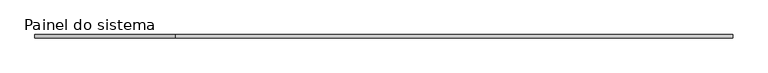
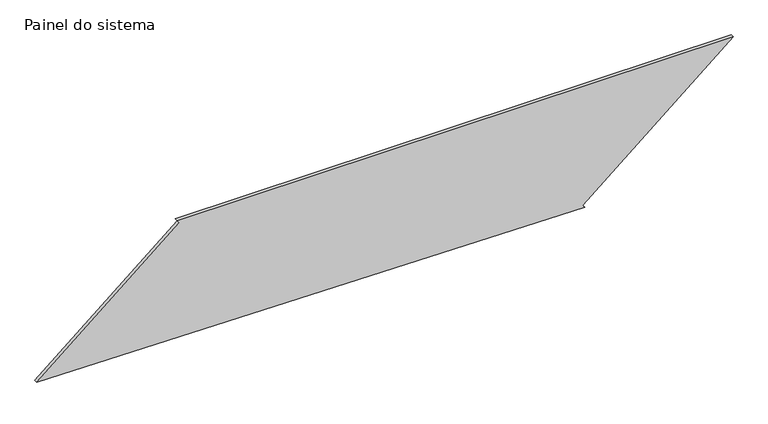
"""IFC4 building model written with IfcOpenShell, lengths in millimetres: plate geometry, Painel do sistema : Envidraçado."""

import ifcopenshell
import ifcopenshell.guid

model = None  # the IFC model being written
_history = None  # IfcOwnerHistory: only IFC2X3 demands one
_inside = {}  # id of a spatial element -> (the spatial element, [elements in it])
_under = {}  # id of a project, library or spatial element -> (it, [spatial elements below it])
_declared = {}  # id of a project -> (the project, [libraries it declares])
_typed = {}  # id of a type object -> (the type object, [elements of that type])
_made_of = {}  # id of a material, layer set ... -> (it, [elements and type objects made of it])


def new_model(schema):
    """Start an empty IFC model of exactly this schema.

    Asked for "IFC4X3", IfcOpenShell would pick the latest addendum, in which some entities
    have other attributes; the version numbers below select the first issue.
    IFC2X3 requires an IfcOwnerHistory on every rooted entity: one is made here for all.
    """
    global model, _history
    if schema == "IFC4X3":
        model = ifcopenshell.file(schema_version=(4, 3, 0, 0))
    else:
        model = ifcopenshell.file(schema=schema)
    _inside.clear()
    _under.clear()
    _declared.clear()
    _typed.clear()
    _made_of.clear()
    _history = None
    if model.schema == "IFC2X3":
        org = make("IfcOrganization", Name="unknown")
        user = make(
            "IfcPersonAndOrganization",
            ThePerson=make("IfcPerson", FamilyName="unknown"),
            TheOrganization=org,
        )
        app = make(
            "IfcApplication",
            ApplicationDeveloper=org,
            Version="unknown",
            ApplicationFullName="unknown",
            ApplicationIdentifier="unknown",
        )
        _history = make(
            "IfcOwnerHistory",
            OwningUser=user,
            OwningApplication=app,
            ChangeAction="ADDED",
            CreationDate=0,
        )
    return model


def make(cls, **values):
    """One entity of the class cls with the attributes given. An attribute that is None is left unset."""
    return model.create_entity(
        cls, **{name: value for name, value in values.items() if value is not None}
    )


def rooted(cls, **values):
    """An entity with a GlobalId (a new one), such as an element, a storey or a relation."""
    return make(cls, GlobalId=ifcopenshell.guid.new(), OwnerHistory=_history, **values)


def si_unit(unit_type, name, prefix=None):
    """IfcSIUnit, for example si_unit("LENGTHUNIT", "METRE", prefix="MILLI")."""
    return make("IfcSIUnit", UnitType=unit_type, Prefix=prefix, Name=name)


def assignment(units):
    """IfcUnitAssignment: the units of a project."""
    return None if units is None else make("IfcUnitAssignment", Units=units)


def point(xyz):
    """IfcCartesianPoint."""
    return None if xyz is None else make("IfcCartesianPoint", Coordinates=xyz)


def direction(xyz):
    """IfcDirection."""
    return None if xyz is None else make("IfcDirection", DirectionRatios=xyz)


def frame(location, z_axis=None, x_axis=None):
    """IfcAxis2Placement3D, a coordinate frame: its origin and axes. An axis left out is left unset."""
    return make(
        "IfcAxis2Placement3D",
        Location=point(location),
        Axis=direction(z_axis),
        RefDirection=direction(x_axis),
    )


def origin():
    """The frame at (0, 0, 0) with its axes left unset."""
    return frame((0.0, 0.0, 0.0))


def place(relative_to, where):
    """IfcLocalPlacement: puts the frame where relative to a parent placement (None: the world)."""
    return make(
        "IfcLocalPlacement", PlacementRelTo=relative_to, RelativePlacement=where
    )


def context(
    kind, dimensions, precision=None, world=None, true_north=None, identifier=None
):
    """IfcGeometricRepresentationContext, for example the 3D "Model" context."""
    return make(
        "IfcGeometricRepresentationContext",
        ContextIdentifier=identifier,
        ContextType=kind,
        CoordinateSpaceDimension=dimensions,
        Precision=precision,
        WorldCoordinateSystem=world,
        TrueNorth=true_north,
    )


def project(units=None, contexts=None):
    """IfcProject with its units and contexts."""
    return rooted(
        "IfcProject",
        Name="project",
        RepresentationContexts=contexts,
        UnitsInContext=assignment(units),
    )


def spatial(cls, under=None, at=None, **own):
    """A site, building, storey or space (cls), placed at a placement, below another one or the project."""
    s = rooted(cls, ObjectPlacement=at, **own)
    if under is not None:
        _under.setdefault(under.id(), (under, []))[1].append(s)
    return s


def polyline(points):
    """IfcPolyline through the points."""
    return make("IfcPolyline", Points=[point(p) for p in points])


def outline(outer, holes=None, kind="AREA"):
    """IfcArbitraryClosedProfileDef: a profile drawn as a closed curve; with holes, ...WithVoids."""
    if holes is None:
        return make("IfcArbitraryClosedProfileDef", ProfileType=kind, OuterCurve=outer)
    return make(
        "IfcArbitraryProfileDefWithVoids",
        ProfileType=kind,
        OuterCurve=outer,
        InnerCurves=holes,
    )


def extrude(swept, where, along, depth):
    """IfcExtrudedAreaSolid: the profile swept, set in the frame where, extruded along a direction by depth."""
    return make(
        "IfcExtrudedAreaSolid",
        SweptArea=swept,
        Position=where,
        ExtrudedDirection=direction(along),
        Depth=depth,
    )


def shape(context_of_items, identifier, shape_type, items):
    """IfcShapeRepresentation: the items that make up one representation, for example the "Body"."""
    return make(
        "IfcShapeRepresentation",
        ContextOfItems=context_of_items,
        RepresentationIdentifier=identifier,
        RepresentationType=shape_type,
        Items=items,
    )


def source(mapping_origin, context_of_items, identifier, shape_type, items):
    """IfcRepresentationMap: a shape defined once, which mapped items show again and again."""
    return make(
        "IfcRepresentationMap",
        MappingOrigin=mapping_origin,
        MappedRepresentation=shape(context_of_items, identifier, shape_type, items),
    )


def transform(
    local_origin,
    x_axis=None,
    y_axis=None,
    z_axis=None,
    scale=None,
    scale2=None,
    scale3=None,
    uniform=True,
):
    """IfcCartesianTransformationOperator3D, or its non-uniform kind. x_axis, y_axis, z_axis: its Axis1, 2, 3."""
    if uniform:
        return make(
            "IfcCartesianTransformationOperator3D",
            Axis1=direction(x_axis),
            Axis2=direction(y_axis),
            LocalOrigin=point(local_origin),
            Scale=scale,
            Axis3=direction(z_axis),
        )
    return make(
        "IfcCartesianTransformationOperator3DnonUniform",
        Axis1=direction(x_axis),
        Axis2=direction(y_axis),
        LocalOrigin=point(local_origin),
        Scale=scale,
        Axis3=direction(z_axis),
        Scale2=scale2,
        Scale3=scale3,
    )


def mapped(mapping_source, mapping_target):
    """IfcMappedItem: shows the shape of a source again, moved by a transform."""
    return make(
        "IfcMappedItem", MappingSource=mapping_source, MappingTarget=mapping_target
    )


def made_of(thing, what):
    """Note that an element or type object is made of a material, layer set ...; save() writes the relation."""
    if what is not None:
        _made_of.setdefault(what.id(), (what, []))[1].append(thing)
    return thing


def element(
    cls,
    number,
    at=None,
    inside=None,
    cuts=None,
    type_object=None,
    material=None,
    context=None,
    identifier="Body",
    shape_type=None,
    held_by="IfcProductDefinitionShape",
    body=None,
    shapes=None,
    **own,
):
    """One element of the class cls, such as IfcWall. Its Tag is "e" and its number.

    at: its placement. inside: the storey or other place that contains it. cuts: it is an
    opening in that element (IfcRelVoidsElement). A single representation is given by context,
    identifier, shape_type and body (its items); several are given by shapes. held_by: the class
    of the entity that holds the representations. save() writes the other relations.
    """
    e = rooted(cls, Tag="e%d" % number, ObjectPlacement=at, **own)
    if body is not None:
        shapes = [shape(context, identifier, shape_type, body)]
    if shapes is not None:
        e.Representation = make(held_by, Representations=shapes)
    if inside is not None:
        _inside.setdefault(inside.id(), (inside, []))[1].append(e)
    if cuts is not None:
        rooted(
            "IfcRelVoidsElement", RelatingBuildingElement=cuts, RelatedOpeningElement=e
        )
    if type_object is not None:
        _typed.setdefault(type_object.id(), (type_object, []))[1].append(e)
    return made_of(e, material)


def aggregate(whole, parts):
    """IfcRelAggregates: a whole, such as a stair, and the parts it consists of."""
    return rooted("IfcRelAggregates", RelatingObject=whole, RelatedObjects=parts)


def save(model, path):
    """Write the relations noted so far, then the file.

    IfcRelAggregates (storeys below a building ...), IfcRelContainedInSpatialStructure (elements
    in a storey), IfcRelDefinesByType, IfcRelAssociatesMaterial and IfcRelDeclares: one each for
    every whole, place, type object, material and project.
    """
    for whole, parts in _under.values():
        aggregate(whole, parts)
    for where, things in _inside.values():
        rooted(
            "IfcRelContainedInSpatialStructure",
            RelatedElements=things,
            RelatingStructure=where,
        )
    for kind, things in _typed.values():
        rooted("IfcRelDefinesByType", RelatedObjects=things, RelatingType=kind)
    for what, things in _made_of.values():
        rooted("IfcRelAssociatesMaterial", RelatedObjects=things, RelatingMaterial=what)
    for by, libraries in _declared.values():
        rooted("IfcRelDeclares", RelatingContext=by, RelatedDefinitions=libraries)
    model.write(path)


def painel_do_sistema_20c5028e(model_context):
    return source(origin(), model_context, "Body", "SweptSolid", [
        extrude(outline(polyline([(0.0, 1430.7714374), (19.2037959, 1414.7647443), (916.8375919, 2491.6877621), (916.8375919, -1487.3179677), (897.633796, -1471.3112747), (47.1325024, -2491.6877621), (0.0, 1430.7714374)])), frame((0.0, 24.5, 0.0), z_axis=(0.0, 1.0, 0.0), x_axis=(0.0, 0.0, 1.0)), (0.0, 0.0, 1.0), 25.0),
    ])


if __name__ == "__main__":
    model = new_model("IFC4")
    model_context = context("Model", 3, world=origin())
    ifc_project = project(units=[si_unit("LENGTHUNIT", "METRE", prefix="MILLI")], contexts=[model_context])
    site = spatial("IfcSite", under=ifc_project)
    building = spatial("IfcBuilding", under=site)
    placement = place(None, origin())
    painel_do_sistema_shape = painel_do_sistema_20c5028e(model_context)
    element("IfcPlate", 1, ObjectType="Painel do sistema : Envidraçado", at=placement, inside=building, context=model_context, shape_type="MappedRepresentation", body=[
        mapped(painel_do_sistema_shape, transform((0.0, 0.0, 0.0), x_axis=(1.0, 0.0, 0.0), y_axis=(0.0, 1.0, 0.0), z_axis=(0.0, 0.0, 1.0))),
    ])
    save(model, "model.ifc")

# Revit data of these elements
# Type "Painel do sistema : Envidraçado"
#   Construction Type Id = "GSP4R"
#   Analytic Construction = "Vidraça única Pilkington 1/8 pol"
#   Visual Light Transmittance = 0.9
#   Solar Heat Gain Coefficient = 0.86
#   Heat Transfer Coefficient (U) = 6.7069 W/(m²·K)
# Element 1 (IfcPlate, "Painel do sistema : Envidraçado")
#   Materials on its faces: "Vidro"
# Materials
#   "Vidro": class "Vidro", colour RGB 0 128 192, transparency 0.9, Description = "Vidro de sílica", Cost = 0
